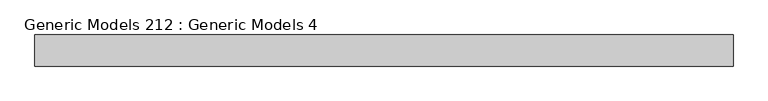
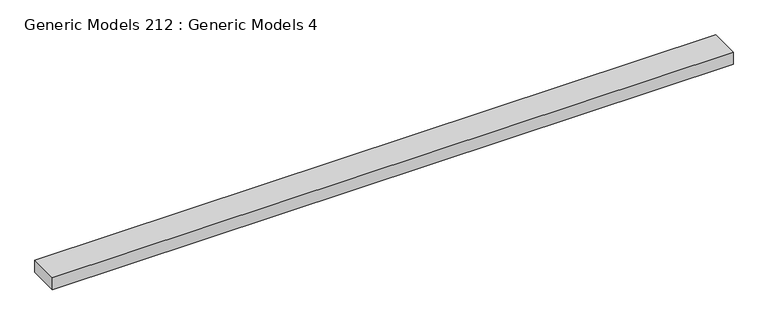
"""IFC4 building model written with IfcOpenShell, lengths in millimetres: proxy geometry, Generic Models 212 : Generic Models 4."""

import ifcopenshell
import ifcopenshell.guid

model = None  # the IFC model being written
_history = None  # IfcOwnerHistory: only IFC2X3 demands one
_inside = {}  # id of a spatial element -> (the spatial element, [elements in it])
_under = {}  # id of a project, library or spatial element -> (it, [spatial elements below it])
_declared = {}  # id of a project -> (the project, [libraries it declares])
_typed = {}  # id of a type object -> (the type object, [elements of that type])
_made_of = {}  # id of a material, layer set ... -> (it, [elements and type objects made of it])


def new_model(schema):
    """Start an empty IFC model of exactly this schema.

    Asked for "IFC4X3", IfcOpenShell would pick the latest addendum, in which some entities
    have other attributes; the version numbers below select the first issue.
    IFC2X3 requires an IfcOwnerHistory on every rooted entity: one is made here for all.
    """
    global model, _history
    if schema == "IFC4X3":
        model = ifcopenshell.file(schema_version=(4, 3, 0, 0))
    else:
        model = ifcopenshell.file(schema=schema)
    _inside.clear()
    _under.clear()
    _declared.clear()
    _typed.clear()
    _made_of.clear()
    _history = None
    if model.schema == "IFC2X3":
        org = make("IfcOrganization", Name="unknown")
        user = make(
            "IfcPersonAndOrganization",
            ThePerson=make("IfcPerson", FamilyName="unknown"),
            TheOrganization=org,
        )
        app = make(
            "IfcApplication",
            ApplicationDeveloper=org,
            Version="unknown",
            ApplicationFullName="unknown",
            ApplicationIdentifier="unknown",
        )
        _history = make(
            "IfcOwnerHistory",
            OwningUser=user,
            OwningApplication=app,
            ChangeAction="ADDED",
            CreationDate=0,
        )
    return model


def make(cls, **values):
    """One entity of the class cls with the attributes given. An attribute that is None is left unset."""
    return model.create_entity(
        cls, **{name: value for name, value in values.items() if value is not None}
    )


def rooted(cls, **values):
    """An entity with a GlobalId (a new one), such as an element, a storey or a relation."""
    return make(cls, GlobalId=ifcopenshell.guid.new(), OwnerHistory=_history, **values)


def si_unit(unit_type, name, prefix=None):
    """IfcSIUnit, for example si_unit("LENGTHUNIT", "METRE", prefix="MILLI")."""
    return make("IfcSIUnit", UnitType=unit_type, Prefix=prefix, Name=name)


def assignment(units):
    """IfcUnitAssignment: the units of a project."""
    return None if units is None else make("IfcUnitAssignment", Units=units)


def point(xyz):
    """IfcCartesianPoint."""
    return None if xyz is None else make("IfcCartesianPoint", Coordinates=xyz)


def direction(xyz):
    """IfcDirection."""
    return None if xyz is None else make("IfcDirection", DirectionRatios=xyz)


def frame(location, z_axis=None, x_axis=None):
    """IfcAxis2Placement3D, a coordinate frame: its origin and axes. An axis left out is left unset."""
    return make(
        "IfcAxis2Placement3D",
        Location=point(location),
        Axis=direction(z_axis),
        RefDirection=direction(x_axis),
    )


def origin():
    """The frame at (0, 0, 0) with its axes left unset."""
    return frame((0.0, 0.0, 0.0))


def place(relative_to, where):
    """IfcLocalPlacement: puts the frame where relative to a parent placement (None: the world)."""
    return make(
        "IfcLocalPlacement", PlacementRelTo=relative_to, RelativePlacement=where
    )


def context(
    kind, dimensions, precision=None, world=None, true_north=None, identifier=None
):
    """IfcGeometricRepresentationContext, for example the 3D "Model" context."""
    return make(
        "IfcGeometricRepresentationContext",
        ContextIdentifier=identifier,
        ContextType=kind,
        CoordinateSpaceDimension=dimensions,
        Precision=precision,
        WorldCoordinateSystem=world,
        TrueNorth=true_north,
    )


def project(units=None, contexts=None):
    """IfcProject with its units and contexts."""
    return rooted(
        "IfcProject",
        Name="project",
        RepresentationContexts=contexts,
        UnitsInContext=assignment(units),
    )


def spatial(cls, under=None, at=None, **own):
    """A site, building, storey or space (cls), placed at a placement, below another one or the project."""
    s = rooted(cls, ObjectPlacement=at, **own)
    if under is not None:
        _under.setdefault(under.id(), (under, []))[1].append(s)
    return s


def polyline(points):
    """IfcPolyline through the points."""
    return make("IfcPolyline", Points=[point(p) for p in points])


def outline(outer, holes=None, kind="AREA"):
    """IfcArbitraryClosedProfileDef: a profile drawn as a closed curve; with holes, ...WithVoids."""
    if holes is None:
        return make("IfcArbitraryClosedProfileDef", ProfileType=kind, OuterCurve=outer)
    return make(
        "IfcArbitraryProfileDefWithVoids",
        ProfileType=kind,
        OuterCurve=outer,
        InnerCurves=holes,
    )


def extrude(swept, where, along, depth):
    """IfcExtrudedAreaSolid: the profile swept, set in the frame where, extruded along a direction by depth."""
    return make(
        "IfcExtrudedAreaSolid",
        SweptArea=swept,
        Position=where,
        ExtrudedDirection=direction(along),
        Depth=depth,
    )


def shape(context_of_items, identifier, shape_type, items):
    """IfcShapeRepresentation: the items that make up one representation, for example the "Body"."""
    return make(
        "IfcShapeRepresentation",
        ContextOfItems=context_of_items,
        RepresentationIdentifier=identifier,
        RepresentationType=shape_type,
        Items=items,
    )


def source(mapping_origin, context_of_items, identifier, shape_type, items):
    """IfcRepresentationMap: a shape defined once, which mapped items show again and again."""
    return make(
        "IfcRepresentationMap",
        MappingOrigin=mapping_origin,
        MappedRepresentation=shape(context_of_items, identifier, shape_type, items),
    )


def transform(
    local_origin,
    x_axis=None,
    y_axis=None,
    z_axis=None,
    scale=None,
    scale2=None,
    scale3=None,
    uniform=True,
):
    """IfcCartesianTransformationOperator3D, or its non-uniform kind. x_axis, y_axis, z_axis: its Axis1, 2, 3."""
    if uniform:
        return make(
            "IfcCartesianTransformationOperator3D",
            Axis1=direction(x_axis),
            Axis2=direction(y_axis),
            LocalOrigin=point(local_origin),
            Scale=scale,
            Axis3=direction(z_axis),
        )
    return make(
        "IfcCartesianTransformationOperator3DnonUniform",
        Axis1=direction(x_axis),
        Axis2=direction(y_axis),
        LocalOrigin=point(local_origin),
        Scale=scale,
        Axis3=direction(z_axis),
        Scale2=scale2,
        Scale3=scale3,
    )


def mapped(mapping_source, mapping_target):
    """IfcMappedItem: shows the shape of a source again, moved by a transform."""
    return make(
        "IfcMappedItem", MappingSource=mapping_source, MappingTarget=mapping_target
    )


def made_of(thing, what):
    """Note that an element or type object is made of a material, layer set ...; save() writes the relation."""
    if what is not None:
        _made_of.setdefault(what.id(), (what, []))[1].append(thing)
    return thing


def element(
    cls,
    number,
    at=None,
    inside=None,
    cuts=None,
    type_object=None,
    material=None,
    context=None,
    identifier="Body",
    shape_type=None,
    held_by="IfcProductDefinitionShape",
    body=None,
    shapes=None,
    **own,
):
    """One element of the class cls, such as IfcWall. Its Tag is "e" and its number.

    at: its placement. inside: the storey or other place that contains it. cuts: it is an
    opening in that element (IfcRelVoidsElement). A single representation is given by context,
    identifier, shape_type and body (its items); several are given by shapes. held_by: the class
    of the entity that holds the representations. save() writes the other relations.
    """
    e = rooted(cls, Tag="e%d" % number, ObjectPlacement=at, **own)
    if body is not None:
        shapes = [shape(context, identifier, shape_type, body)]
    if shapes is not None:
        e.Representation = make(held_by, Representations=shapes)
    if inside is not None:
        _inside.setdefault(inside.id(), (inside, []))[1].append(e)
    if cuts is not None:
        rooted(
            "IfcRelVoidsElement", RelatingBuildingElement=cuts, RelatedOpeningElement=e
        )
    if type_object is not None:
        _typed.setdefault(type_object.id(), (type_object, []))[1].append(e)
    return made_of(e, material)


def aggregate(whole, parts):
    """IfcRelAggregates: a whole, such as a stair, and the parts it consists of."""
    return rooted("IfcRelAggregates", RelatingObject=whole, RelatedObjects=parts)


def save(model, path):
    """Write the relations noted so far, then the file.

    IfcRelAggregates (storeys below a building ...), IfcRelContainedInSpatialStructure (elements
    in a storey), IfcRelDefinesByType, IfcRelAssociatesMaterial and IfcRelDeclares: one each for
    every whole, place, type object, material and project.
    """
    for whole, parts in _under.values():
        aggregate(whole, parts)
    for where, things in _inside.values():
        rooted(
            "IfcRelContainedInSpatialStructure",
            RelatedElements=things,
            RelatingStructure=where,
        )
    for kind, things in _typed.values():
        rooted("IfcRelDefinesByType", RelatedObjects=things, RelatingType=kind)
    for what, things in _made_of.values():
        rooted("IfcRelAssociatesMaterial", RelatedObjects=things, RelatingMaterial=what)
    for by, libraries in _declared.values():
        rooted("IfcRelDeclares", RelatingContext=by, RelatedDefinitions=libraries)
    model.write(path)


def generic_models_212_generic_models_4_de7b88a7(model_context):
    return source(origin(), model_context, "Body", "SweptSolid", [
        extrude(outline(polyline([(8409.0828684, 11302.4269662), (8409.0828684, 10471.9172159), (-10234.5171316, 10471.9172159), (-10234.5171316, 11302.4269662), (8409.0828684, 11302.4269662)])), frame((0.0, 0.0, 126402.846), z_axis=(0.0, 0.0, 1.0), x_axis=(1.0, 0.0, 0.0)), (0.0, 0.0, 1.0), 347.5929632),
    ])


if __name__ == "__main__":
    model = new_model("IFC4")
    model_context = context("Model", 3, world=origin())
    ifc_project = project(units=[si_unit("LENGTHUNIT", "METRE", prefix="MILLI")], contexts=[model_context])
    site = spatial("IfcSite", under=ifc_project)
    building = spatial("IfcBuilding", under=site)
    placement = place(None, origin())
    generic_models_212_generic_models_4_shape = generic_models_212_generic_models_4_de7b88a7(model_context)
    element("IfcBuildingElementProxy", 1, Name="Generic Models 212 : Generic Models 4", ObjectType="Generic Models 212 : Generic Models 4", at=placement, inside=building, context=model_context, shape_type="MappedRepresentation", body=[
        mapped(generic_models_212_generic_models_4_shape, transform((0.0, 0.0, 0.0), x_axis=(1.0, 0.0, 0.0), y_axis=(0.0, 1.0, 0.0), z_axis=(0.0, 0.0, 1.0))),
    ])
    save(model, "model.ifc")

# Revit data of these elements
# Element 1 (IfcBuildingElementProxy, "Generic Models 212 : Generic Models 4")
#   Materials on its faces: "_BATT INSUL. (R-FACTOR = R38 MIN) OVER CLASS II VAPOR RETARDER(TOWARD INTERIOR)"
# Materials
#   "_BATT INSUL. (R-FACTOR = R38 MIN) OVER CLASS II VAPOR RETARDER(TOWARD INTERIOR)": class "Generic", colour RGB 227 210 251, transparency 0, Cost = 0
